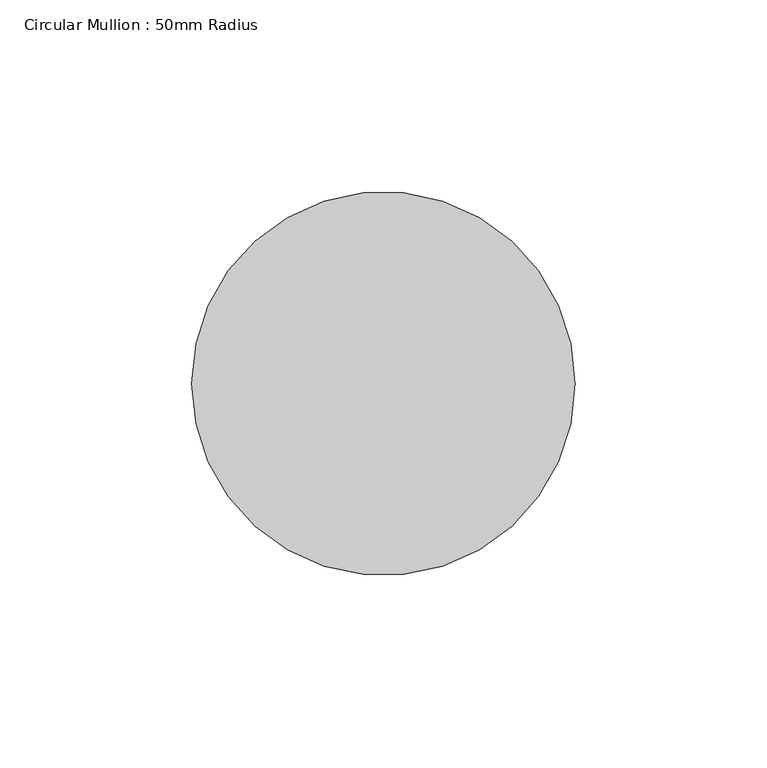
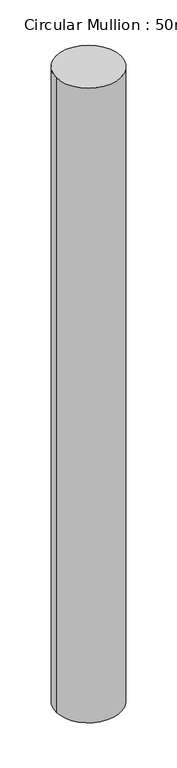
"""IFC4 building model written with IfcOpenShell, lengths in millimetres: member geometry, Circular Mullion : 50mm Radius."""

from ifc_helpers import new_model, si_unit, point, frame, origin, origin_2d, place, context, project, spatial, circle_curve, trimmed, segment, composite_curve, outline, extrude, source, transform, mapped, element, save


def circular_mullion_50mm_radius_9398a81e(model_context):
    return source(origin(), model_context, "Body", "SweptSolid", [
        extrude(outline(composite_curve([segment(trimmed(circle_curve(origin_2d(), 50.0), [point((50.0, 0.0))], [point((-50.0, 0.0))], False, "CARTESIAN"), True, "CONTINUOUS"), segment(trimmed(circle_curve(origin_2d(), 50.0), [point((-50.0, 0.0))], [point((50.0, 0.0))], False, "CARTESIAN"), True, "CONTINUOUS")], self_intersect=False)), frame((0.0, 0.0, -1036.0589268), z_axis=(0.0, 0.0, 1.0), x_axis=(1.0, 0.0, 0.0)), (0.0, 0.0, 1.0), 1036.0589268),
    ])


if __name__ == "__main__":
    model = new_model("IFC4")
    model_context = context("Model", 3, world=origin())
    ifc_project = project(units=[si_unit("LENGTHUNIT", "METRE", prefix="MILLI")], contexts=[model_context])
    site = spatial("IfcSite", under=ifc_project)
    building = spatial("IfcBuilding", under=site)
    placement = place(None, origin())
    circular_mullion_50mm_radius_shape = circular_mullion_50mm_radius_9398a81e(model_context)
    element("IfcMember", 1, ObjectType="Circular Mullion : 50mm Radius", at=placement, inside=building, context=model_context, shape_type="MappedRepresentation", body=[
        mapped(circular_mullion_50mm_radius_shape, transform((0.0, 0.0, 0.0), x_axis=(1.0, 0.0, 0.0), y_axis=(0.0, 1.0, 0.0), z_axis=(0.0, 0.0, 1.0))),
    ])
    save(model, "model.ifc")

# Revit data of these elements
# Type "Circular Mullion : 50mm Radius"
#   built-in parameter 1007350 = 0.164042 (stored number, unit not read)
# Element 1 (IfcMember, "Circular Mullion : 50mm Radius")
#   Materials on its faces: "Aluminium"
# Materials
#   "Aluminium": class "Metal", colour RGB 247 247 247, transparency 0, Description = "Aluminium 6061", Cost = 0
